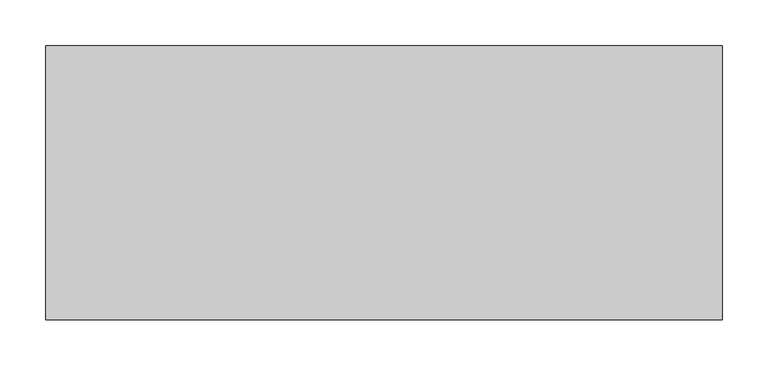
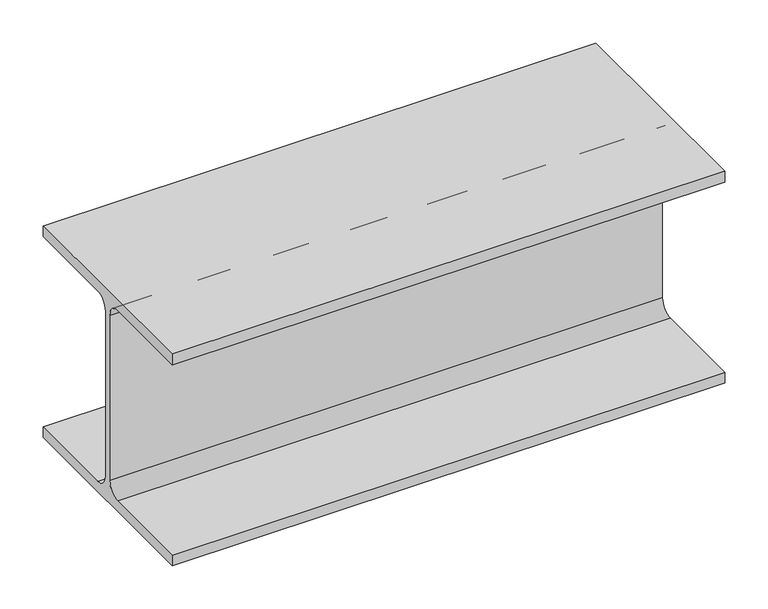
"""IFC4 building model written with IfcOpenShell, lengths in millimetres: beam geometry, 0912_Steel Framing_H-KSD3502 : H_SB_ASB_H-300x300x10x15."""

from ifc_helpers import new_model, si_unit, point, frame, frame_2d, origin, place, context, project, spatial, polyline, circle_curve, trimmed, segment, composite_curve, outline, extrude, source, transform, mapped, element, save


def beam_3840d5b5(model_context):
    return source(origin(), model_context, "Body", "SweptSolid", [
        extrude(outline(composite_curve([segment(polyline([(150.0, -135.0), (150.0, -150.0), (-150.0, -150.0), (-150.0, -135.0), (-23.0, -135.0)]), True, "CONTINUOUS"), segment(trimmed(circle_curve(frame_2d((-23.0, -117.0)), 18.0), [point((-23.0, -135.0))], [point((-5.0, -117.0))], True, "CARTESIAN"), True, "CONTINUOUS"), segment(polyline([(-5.0, -117.0), (-5.0, 117.0)]), True, "CONTINUOUS"), segment(trimmed(circle_curve(frame_2d((-23.0, 117.0)), 18.0), [point((-5.0, 117.0))], [point((-23.0, 135.0))], True, "CARTESIAN"), True, "CONTINUOUS"), segment(polyline([(-23.0, 135.0), (-150.0, 135.0), (-150.0, 150.0), (150.0, 150.0), (150.0, 135.0), (23.0, 135.0)]), True, "CONTINUOUS"), segment(trimmed(circle_curve(frame_2d((23.0, 117.0)), 18.0), [point((23.0, 135.0))], [point((5.0, 117.0))], True, "CARTESIAN"), True, "CONTINUOUS"), segment(polyline([(5.0, 117.0), (5.0, -117.0)]), True, "CONTINUOUS"), segment(trimmed(circle_curve(frame_2d((23.0, -117.0)), 18.0), [point((5.0, -117.0))], [point((23.0, -135.0))], True, "CARTESIAN"), True, "CONTINUOUS"), segment(polyline([(23.0, -135.0), (150.0, -135.0)]), True, "CONTINUOUS")], self_intersect=False)), frame((-237.9749298, 0.0, 0.0), z_axis=(1.0, 0.0, 0.0), x_axis=(0.0, 1.0, 0.0)), (0.0, 0.0, 1.0), 740.4687108),
    ])


if __name__ == "__main__":
    model = new_model("IFC4")
    model_context = context("Model", 3, world=origin())
    ifc_project = project(units=[si_unit("LENGTHUNIT", "METRE", prefix="MILLI")], contexts=[model_context])
    site = spatial("IfcSite", under=ifc_project)
    building = spatial("IfcBuilding", under=site)
    placement = place(None, origin())
    beam_shape = beam_3840d5b5(model_context)
    element("IfcBeam", 1, ObjectType="0912_Steel Framing_H-KSD3502 : H_SB_ASB_H-300x300x10x15", at=placement, inside=building, context=model_context, shape_type="MappedRepresentation", body=[
        mapped(beam_shape, transform((0.0, 0.0, 0.0), x_axis=(1.0, 0.0, 0.0), y_axis=(0.0, 1.0, 0.0), z_axis=(0.0, 0.0, 1.0))),
    ])
    save(model, "model.ifc")

# Revit data of these elements
# Type "0912_Steel Framing_H-KSD3502 : H_SB_ASB_H-300x300x10x15"
#   H_WM Code_1 = "S01AA001-00001 | Main Steel Structure Fabrication Work | Shelter/Building | Heavy Steel - Standard (Weight≥90KG/M) | Material: (   )"
#   H_WM Code_2 = "S03AA027-00001 | Main Steel Structure Erection Work | Shelter/Building | Heavy Steel (Weight≥90KG/M) | Material: (   )"
#   H_WM Code_3 = "S01AA010-00001 | Main Steel Structure Fabrication Work | Shelter/Building | Steel Painting/Coating | for Non-Fireproofed Steel Surface, Surface Preparation, Primer, Second & Final Coat | Material: (   )"
#   H_Q'ty Cal Type Tag = "SB-Q2"
#   Width = 30.0 cm
#   Web Thickness = 1.0 cm
#   Web Fillet = 1.8 cm
#   Warping Constant = 1370000.0 cm⁶
#   W = 0
#   Torsional Moment of Inertia = 77.00 cm⁴
#   Section Area = 119.8 cm²
#   Plastic Modulus weak axis = 684.0 cm³
#   Plastic Modulus strong axis = 1500.0 cm³
#   Perimeter = 1.75 m²/m
#   Nominal Weight = 94.00 kgf/m
#   Moment of Inertia weak axis = 6750.00 cm⁴
#   Moment of Inertia strong axis = 20400.00 cm⁴
#   Height = 30.0 cm
#   Flange Thickness = 1.5 cm
#   Elastic Modulus weak axis = 450.0 cm³
#   Elastic Modulus strong axis = 1360.0 cm³
#   Centroid Vertical = 15.0 cm
#   Centroid Horizontal = 15.0 cm
#   Ix = 204000000
#   Length [instance default] = 1.5240 m
#   Zx = 1500000
#   b = 0.3000 m
#   h = 0.3000 m
#   r = 0.0180 m
#   s = 0.0100 m
#   t = 0.0150 m
#   A = 0.01198 m²
#   Structural Material [instance default] = Steel, 45-345
#   Assembly Code = ""
# Element 1 (IfcBeam, "0912_Steel Framing_H-KSD3502 : H_SB_ASB_H-300x300x10x15")
#   Structural Material = none
# Materials
#   "Steel, 45-345": class "Metal", colour RGB 189 187 185, transparency 0, Description = "Steel 345 MPa", Cost = 0
